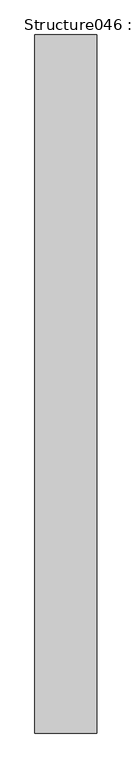
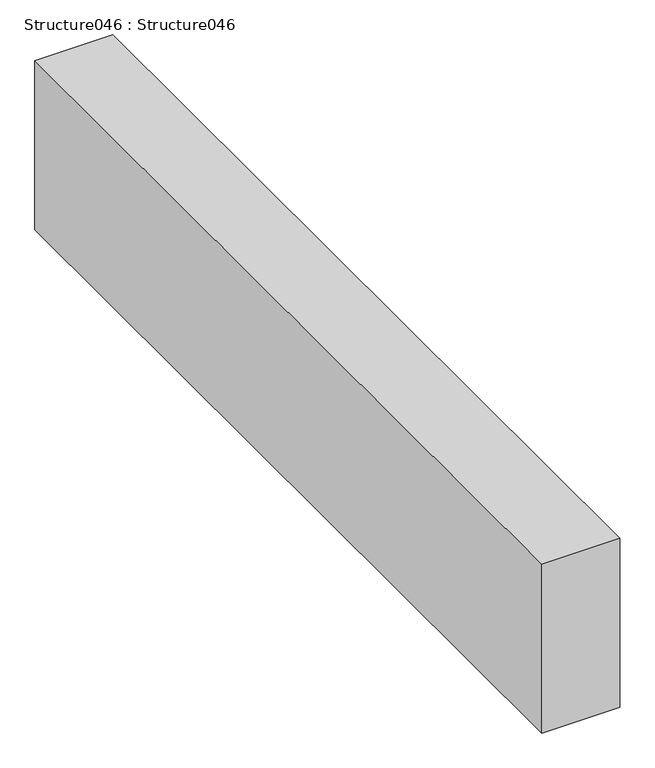
"""IFC4 building model written with IfcOpenShell, lengths in millimetres: proxy geometry, Structure046 : Structure046."""

import ifcopenshell
import ifcopenshell.guid

model = None  # the IFC model being written
_history = None  # IfcOwnerHistory: only IFC2X3 demands one
_inside = {}  # id of a spatial element -> (the spatial element, [elements in it])
_under = {}  # id of a project, library or spatial element -> (it, [spatial elements below it])
_declared = {}  # id of a project -> (the project, [libraries it declares])
_typed = {}  # id of a type object -> (the type object, [elements of that type])
_made_of = {}  # id of a material, layer set ... -> (it, [elements and type objects made of it])


def new_model(schema):
    """Start an empty IFC model of exactly this schema.

    Asked for "IFC4X3", IfcOpenShell would pick the latest addendum, in which some entities
    have other attributes; the version numbers below select the first issue.
    IFC2X3 requires an IfcOwnerHistory on every rooted entity: one is made here for all.
    """
    global model, _history
    if schema == "IFC4X3":
        model = ifcopenshell.file(schema_version=(4, 3, 0, 0))
    else:
        model = ifcopenshell.file(schema=schema)
    _inside.clear()
    _under.clear()
    _declared.clear()
    _typed.clear()
    _made_of.clear()
    _history = None
    if model.schema == "IFC2X3":
        org = make("IfcOrganization", Name="unknown")
        user = make(
            "IfcPersonAndOrganization",
            ThePerson=make("IfcPerson", FamilyName="unknown"),
            TheOrganization=org,
        )
        app = make(
            "IfcApplication",
            ApplicationDeveloper=org,
            Version="unknown",
            ApplicationFullName="unknown",
            ApplicationIdentifier="unknown",
        )
        _history = make(
            "IfcOwnerHistory",
            OwningUser=user,
            OwningApplication=app,
            ChangeAction="ADDED",
            CreationDate=0,
        )
    return model


def make(cls, **values):
    """One entity of the class cls with the attributes given. An attribute that is None is left unset."""
    return model.create_entity(
        cls, **{name: value for name, value in values.items() if value is not None}
    )


def rooted(cls, **values):
    """An entity with a GlobalId (a new one), such as an element, a storey or a relation."""
    return make(cls, GlobalId=ifcopenshell.guid.new(), OwnerHistory=_history, **values)


def si_unit(unit_type, name, prefix=None):
    """IfcSIUnit, for example si_unit("LENGTHUNIT", "METRE", prefix="MILLI")."""
    return make("IfcSIUnit", UnitType=unit_type, Prefix=prefix, Name=name)


def assignment(units):
    """IfcUnitAssignment: the units of a project."""
    return None if units is None else make("IfcUnitAssignment", Units=units)


def point(xyz):
    """IfcCartesianPoint."""
    return None if xyz is None else make("IfcCartesianPoint", Coordinates=xyz)


def direction(xyz):
    """IfcDirection."""
    return None if xyz is None else make("IfcDirection", DirectionRatios=xyz)


def frame(location, z_axis=None, x_axis=None):
    """IfcAxis2Placement3D, a coordinate frame: its origin and axes. An axis left out is left unset."""
    return make(
        "IfcAxis2Placement3D",
        Location=point(location),
        Axis=direction(z_axis),
        RefDirection=direction(x_axis),
    )


def origin():
    """The frame at (0, 0, 0) with its axes left unset."""
    return frame((0.0, 0.0, 0.0))


def place(relative_to, where):
    """IfcLocalPlacement: puts the frame where relative to a parent placement (None: the world)."""
    return make(
        "IfcLocalPlacement", PlacementRelTo=relative_to, RelativePlacement=where
    )


def context(
    kind, dimensions, precision=None, world=None, true_north=None, identifier=None
):
    """IfcGeometricRepresentationContext, for example the 3D "Model" context."""
    return make(
        "IfcGeometricRepresentationContext",
        ContextIdentifier=identifier,
        ContextType=kind,
        CoordinateSpaceDimension=dimensions,
        Precision=precision,
        WorldCoordinateSystem=world,
        TrueNorth=true_north,
    )


def project(units=None, contexts=None):
    """IfcProject with its units and contexts."""
    return rooted(
        "IfcProject",
        Name="project",
        RepresentationContexts=contexts,
        UnitsInContext=assignment(units),
    )


def spatial(cls, under=None, at=None, **own):
    """A site, building, storey or space (cls), placed at a placement, below another one or the project."""
    s = rooted(cls, ObjectPlacement=at, **own)
    if under is not None:
        _under.setdefault(under.id(), (under, []))[1].append(s)
    return s


def polyline(points):
    """IfcPolyline through the points."""
    return make("IfcPolyline", Points=[point(p) for p in points])


def outline(outer, holes=None, kind="AREA"):
    """IfcArbitraryClosedProfileDef: a profile drawn as a closed curve; with holes, ...WithVoids."""
    if holes is None:
        return make("IfcArbitraryClosedProfileDef", ProfileType=kind, OuterCurve=outer)
    return make(
        "IfcArbitraryProfileDefWithVoids",
        ProfileType=kind,
        OuterCurve=outer,
        InnerCurves=holes,
    )


def extrude(swept, where, along, depth):
    """IfcExtrudedAreaSolid: the profile swept, set in the frame where, extruded along a direction by depth."""
    return make(
        "IfcExtrudedAreaSolid",
        SweptArea=swept,
        Position=where,
        ExtrudedDirection=direction(along),
        Depth=depth,
    )


def shape(context_of_items, identifier, shape_type, items):
    """IfcShapeRepresentation: the items that make up one representation, for example the "Body"."""
    return make(
        "IfcShapeRepresentation",
        ContextOfItems=context_of_items,
        RepresentationIdentifier=identifier,
        RepresentationType=shape_type,
        Items=items,
    )


def source(mapping_origin, context_of_items, identifier, shape_type, items):
    """IfcRepresentationMap: a shape defined once, which mapped items show again and again."""
    return make(
        "IfcRepresentationMap",
        MappingOrigin=mapping_origin,
        MappedRepresentation=shape(context_of_items, identifier, shape_type, items),
    )


def transform(
    local_origin,
    x_axis=None,
    y_axis=None,
    z_axis=None,
    scale=None,
    scale2=None,
    scale3=None,
    uniform=True,
):
    """IfcCartesianTransformationOperator3D, or its non-uniform kind. x_axis, y_axis, z_axis: its Axis1, 2, 3."""
    if uniform:
        return make(
            "IfcCartesianTransformationOperator3D",
            Axis1=direction(x_axis),
            Axis2=direction(y_axis),
            LocalOrigin=point(local_origin),
            Scale=scale,
            Axis3=direction(z_axis),
        )
    return make(
        "IfcCartesianTransformationOperator3DnonUniform",
        Axis1=direction(x_axis),
        Axis2=direction(y_axis),
        LocalOrigin=point(local_origin),
        Scale=scale,
        Axis3=direction(z_axis),
        Scale2=scale2,
        Scale3=scale3,
    )


def mapped(mapping_source, mapping_target):
    """IfcMappedItem: shows the shape of a source again, moved by a transform."""
    return make(
        "IfcMappedItem", MappingSource=mapping_source, MappingTarget=mapping_target
    )


def made_of(thing, what):
    """Note that an element or type object is made of a material, layer set ...; save() writes the relation."""
    if what is not None:
        _made_of.setdefault(what.id(), (what, []))[1].append(thing)
    return thing


def element(
    cls,
    number,
    at=None,
    inside=None,
    cuts=None,
    type_object=None,
    material=None,
    context=None,
    identifier="Body",
    shape_type=None,
    held_by="IfcProductDefinitionShape",
    body=None,
    shapes=None,
    **own,
):
    """One element of the class cls, such as IfcWall. Its Tag is "e" and its number.

    at: its placement. inside: the storey or other place that contains it. cuts: it is an
    opening in that element (IfcRelVoidsElement). A single representation is given by context,
    identifier, shape_type and body (its items); several are given by shapes. held_by: the class
    of the entity that holds the representations. save() writes the other relations.
    """
    e = rooted(cls, Tag="e%d" % number, ObjectPlacement=at, **own)
    if body is not None:
        shapes = [shape(context, identifier, shape_type, body)]
    if shapes is not None:
        e.Representation = make(held_by, Representations=shapes)
    if inside is not None:
        _inside.setdefault(inside.id(), (inside, []))[1].append(e)
    if cuts is not None:
        rooted(
            "IfcRelVoidsElement", RelatingBuildingElement=cuts, RelatedOpeningElement=e
        )
    if type_object is not None:
        _typed.setdefault(type_object.id(), (type_object, []))[1].append(e)
    return made_of(e, material)


def aggregate(whole, parts):
    """IfcRelAggregates: a whole, such as a stair, and the parts it consists of."""
    return rooted("IfcRelAggregates", RelatingObject=whole, RelatedObjects=parts)


def save(model, path):
    """Write the relations noted so far, then the file.

    IfcRelAggregates (storeys below a building ...), IfcRelContainedInSpatialStructure (elements
    in a storey), IfcRelDefinesByType, IfcRelAssociatesMaterial and IfcRelDeclares: one each for
    every whole, place, type object, material and project.
    """
    for whole, parts in _under.values():
        aggregate(whole, parts)
    for where, things in _inside.values():
        rooted(
            "IfcRelContainedInSpatialStructure",
            RelatedElements=things,
            RelatingStructure=where,
        )
    for kind, things in _typed.values():
        rooted("IfcRelDefinesByType", RelatedObjects=things, RelatingType=kind)
    for what, things in _made_of.values():
        rooted("IfcRelAssociatesMaterial", RelatedObjects=things, RelatingMaterial=what)
    for by, libraries in _declared.values():
        rooted("IfcRelDeclares", RelatingContext=by, RelatedDefinitions=libraries)
    model.write(path)


def structure046_structure046_5e824010(model_context):
    return source(origin(), model_context, "Body", "SweptSolid", [
        extrude(outline(polyline([(-2303.2114422, -1052.8906574), (-2481.0114422, -1052.8906574), (-2481.0114422, 947.1093426), (-2303.2114422, 947.1093426), (-2303.2114422, -1052.8906574)])), frame((0.0, 0.0, 39706.296), z_axis=(0.0, 0.0, 1.0), x_axis=(1.0, 0.0, 0.0)), (0.0, 0.0, 1.0), 406.4),
    ])


if __name__ == "__main__":
    model = new_model("IFC4")
    model_context = context("Model", 3, world=origin())
    ifc_project = project(units=[si_unit("LENGTHUNIT", "METRE", prefix="MILLI")], contexts=[model_context])
    site = spatial("IfcSite", under=ifc_project)
    building = spatial("IfcBuilding", under=site)
    placement = place(None, origin())
    structure046_structure046_shape = structure046_structure046_5e824010(model_context)
    element("IfcBuildingElementProxy", 1, Name="Structure046 : Structure046", ObjectType="Structure046 : Structure046", at=placement, inside=building, context=model_context, shape_type="MappedRepresentation", body=[
        mapped(structure046_structure046_shape, transform((0.0, 0.0, 0.0), x_axis=(1.0, 0.0, 0.0), y_axis=(0.0, 1.0, 0.0), z_axis=(0.0, 0.0, 1.0))),
    ])
    save(model, "model.ifc")

# Revit data of these elements
# Type "Structure046 : Structure046"
#   NameOverride = "Structure046"
# Element 1 (IfcBuildingElementProxy, "Structure046 : Structure046")
#   Materials on its faces: "STRUCTURAL MEMBER (SEE DWGS)"
# Materials
#   "STRUCTURAL MEMBER (SEE DWGS)": class "Unassigned", colour RGB 214 178 158, transparency 0, Cost = 0
